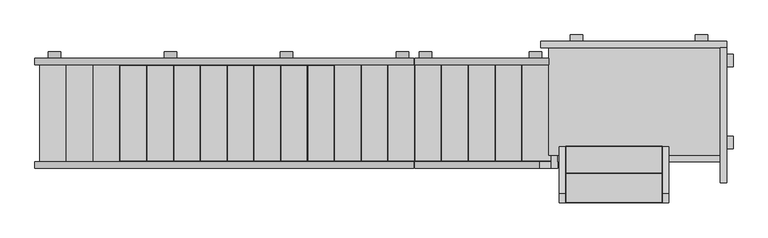
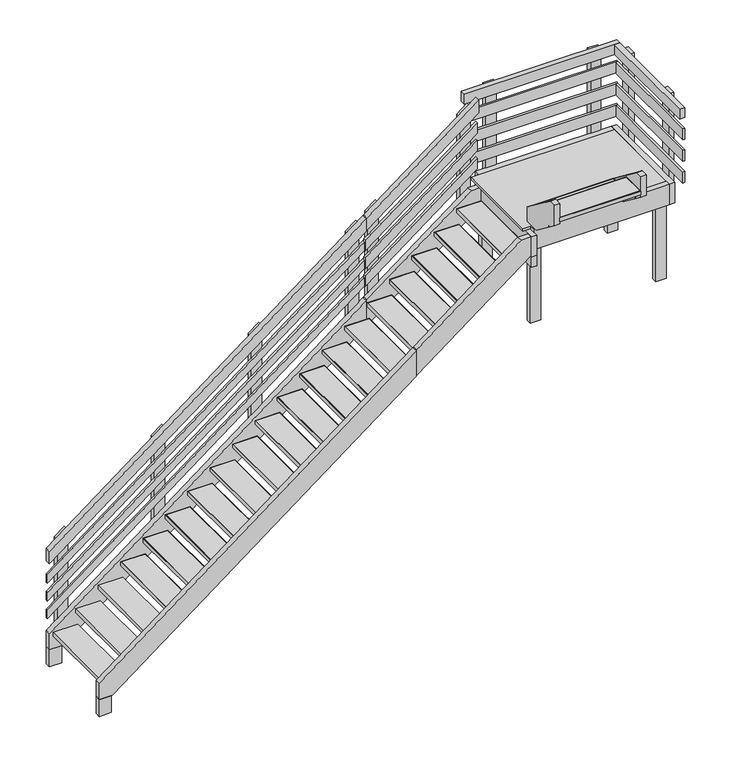
"""IFC4 building model written with IfcOpenShell, lengths in millimetres: stair geometry, Treppen : Treppen."""

from ifc_helpers import new_model, si_unit, frame, origin, place, context, project, spatial, polyline, outline, extrude, faceted_brep, source, transform, mapped, element, save


def stair_8a71ca67(model_context):
    return source(origin(), model_context, "Body", "SolidModel", [
        extrude(outline(polyline([(12040.927184, 9252.4494152), (12100.927184, 9252.4494152), (12100.927184, 9136.4494152), (12040.927184, 9136.4494152), (12040.927184, 9252.4494152)])), frame((0.0, 0.0, 3202.113), z_axis=(0.0, 0.0, 1.0), x_axis=(1.0, 0.0, 0.0)), (0.0, 0.0, 1.0), 1210.0),
        extrude(outline(polyline([(12040.927184, 10019.5272422), (12100.927184, 10019.5272422), (12100.927184, 9903.5272422), (12040.927184, 9903.5272422), (12040.927184, 10019.5272422)])), frame((0.0, 0.0, 3202.113), z_axis=(0.0, 0.0, 1.0), x_axis=(1.0, 0.0, 0.0)), (0.0, 0.0, 1.0), 1210.0),
        extrude(outline(polyline([(11748.927284, 10199.5272422), (11864.927284, 10199.5272422), (11864.927284, 10139.5272422), (11748.927284, 10139.5272422), (11748.927284, 10199.5272422)])), frame((0.0, 0.0, 3202.113), z_axis=(0.0, 0.0, 1.0), x_axis=(1.0, 0.0, 0.0)), (0.0, 0.0, 1.0), 1210.0),
        extrude(outline(polyline([(10580.970284, 10199.5272422), (10696.970284, 10199.5272422), (10696.970284, 10139.5272422), (10580.970284, 10139.5272422), (10580.970284, 10199.5272422)])), frame((0.0, 0.0, 3202.113), z_axis=(0.0, 0.0, 1.0), x_axis=(1.0, 0.0, 0.0)), (0.0, 0.0, 1.0), 1210.0),
        extrude(outline(polyline([(3061.4008007, 10198.6231113), (3149.5608007, 10314.6231113), (4355.2057254, 10314.6231113), (4267.0457213, 10198.6231113), (3061.4008007, 10198.6231113)])), frame((0.0, 9982.5272422, 0.0), z_axis=(0.0, 1.0, 0.0), x_axis=(0.0, 0.0, 1.0)), (0.0, 0.0, 1.0), 60.0),
        extrude(outline(polyline([(2282.7992976, 9174.1474494), (2370.9592976, 9290.1474494), (3576.6042224, 9290.1474494), (3488.4442183, 9174.1474494), (2282.7992976, 9174.1474494)])), frame((0.0, 9982.5272422, 0.0), z_axis=(0.0, 1.0, 0.0), x_axis=(0.0, 0.0, 1.0)), (0.0, 0.0, 1.0), 60.0),
        extrude(outline(polyline([(2118.4713054, 8957.926407), (2206.6313054, 9073.926407), (3412.2762301, 9073.926407), (3324.116226, 8957.926407), (2118.4713054, 8957.926407)])), frame((0.0, 9982.5272422, 0.0), z_axis=(0.0, 1.0, 0.0), x_axis=(0.0, 0.0, 1.0)), (0.0, 0.0, 1.0), 60.0),
        extrude(outline(polyline([(1295.3913054, 7874.926407), (1383.5513054, 7990.926407), (2589.1962301, 7990.926407), (2501.036226, 7874.926407), (1295.3913054, 7874.926407)])), frame((0.0, 9982.5272422, 0.0), z_axis=(0.0, 1.0, 0.0), x_axis=(0.0, 0.0, 1.0)), (0.0, 0.0, 1.0), 60.0),
        extrude(outline(polyline([(472.3113054, 6791.926407), (560.4713054, 6907.926407), (1766.1162301, 6907.926407), (1677.956226, 6791.926407), (472.3113054, 6791.926407)])), frame((0.0, 9982.5272422, 0.0), z_axis=(0.0, 1.0, 0.0), x_axis=(0.0, 0.0, 1.0)), (0.0, 0.0, 1.0), 60.0),
        extrude(outline(polyline([(-350.7686946, 5708.926407), (-262.6086946, 5824.926407), (943.036192, 5824.926407), (854.8761879, 5708.926407), (-350.7686946, 5708.926407)])), frame((0.0, 9982.5272422, 0.0), z_axis=(0.0, 1.0, 0.0), x_axis=(0.0, 0.0, 1.0)), (0.0, 0.0, 1.0), 60.0),
        extrude(outline(polyline([(12016.927184, 10115.5272422), (12040.927184, 10115.5272422), (12040.927184, 8819.5272422), (12016.927184, 8819.5272422), (12016.927184, 10115.5272422)])), frame((0.0, 0.0, 4072.113), z_axis=(0.0, 0.0, 1.0), x_axis=(1.0, 0.0, 0.0)), (0.0, 0.0, 1.0), 130.0),
        extrude(outline(polyline([(12016.927184, 10115.5272422), (12040.927184, 10115.5272422), (12040.927184, 8819.5272422), (12016.927184, 8819.5272422), (12016.927184, 10115.5272422)])), frame((0.0, 0.0, 3817.113), z_axis=(0.0, 0.0, 1.0), x_axis=(1.0, 0.0, 0.0)), (0.0, 0.0, 1.0), 130.0),
        extrude(outline(polyline([(12016.927184, 10115.5272422), (12040.927184, 10115.5272422), (12040.927184, 8819.5272422), (12016.927184, 8819.5272422), (12016.927184, 10115.5272422)])), frame((0.0, 0.0, 3562.113), z_axis=(0.0, 0.0, 1.0), x_axis=(1.0, 0.0, 0.0)), (0.0, 0.0, 1.0), 130.0),
        extrude(outline(polyline([(11980.927184, 10079.5272422), (12040.927184, 10079.5272422), (12040.927184, 8819.5272422), (11980.927184, 8819.5272422), (11980.927184, 10079.5272422)])), frame((0.0, 0.0, 4327.113), z_axis=(0.0, 0.0, 1.0), x_axis=(1.0, 0.0, 0.0)), (0.0, 0.0, 1.0), 116.0),
        extrude(outline(polyline([(10307.870484, 10139.5272422), (12040.927184, 10139.5272422), (12040.927184, 10115.5272422), (10307.870484, 10115.5272422), (10307.870484, 10139.5272422)])), frame((0.0, 0.0, 3562.113), z_axis=(0.0, 0.0, 1.0), x_axis=(1.0, 0.0, 0.0)), (0.0, 0.0, 1.0), 130.0),
        extrude(outline(polyline([(10307.870484, 10139.5272422), (12040.927184, 10139.5272422), (12040.927184, 10115.5272422), (10307.870484, 10115.5272422), (10307.870484, 10139.5272422)])), frame((0.0, 0.0, 3817.113), z_axis=(0.0, 0.0, 1.0), x_axis=(1.0, 0.0, 0.0)), (0.0, 0.0, 1.0), 130.0),
        extrude(outline(polyline([(10307.870484, 10139.5272422), (12040.927184, 10139.5272422), (12040.927184, 10115.5272422), (10307.870484, 10115.5272422), (10307.870484, 10139.5272422)])), frame((0.0, 0.0, 4072.113), z_axis=(0.0, 0.0, 1.0), x_axis=(1.0, 0.0, 0.0)), (0.0, 0.0, 1.0), 130.0),
        extrude(outline(polyline([(402.0866128, 5585.8451154), (3087.6090608, 9119.4271203), (3188.091099, 9119.4271181), (502.568651, 5585.8451132), (402.0866128, 5585.8451154)])), frame((0.0, 9958.5272422, 0.0), z_axis=(0.0, 1.0, 0.0), x_axis=(0.0, 0.0, 1.0)), (0.0, 0.0, 1.0), 24.0),
        extrude(outline(polyline([(2978.466099, 9119.4271181), (292.943651, 5585.8451132), (192.4616128, 5585.8451154), (2877.9840608, 9119.4271203), (2978.466099, 9119.4271181)])), frame((0.0, 9958.5272422, 0.0), z_axis=(0.0, 1.0, 0.0), x_axis=(0.0, 0.0, 1.0)), (0.0, 0.0, 1.0), 24.0),
        extrude(outline(polyline([(2768.841199, 9119.4271181), (83.318751, 5585.8451132), (-17.1632872, 5585.8451154), (2668.3591608, 9119.4271203), (2768.841199, 9119.4271181)])), frame((0.0, 9958.5272422, 0.0), z_axis=(0.0, 1.0, 0.0), x_axis=(0.0, 0.0, 1.0)), (0.0, 0.0, 1.0), 24.0),
        extrude(outline(polyline([(4158.2512383, 10379.427087), (3208.2512387, 9129.4271455), (3082.648691, 9129.4271483), (4032.6486905, 10379.4270898), (4158.2512383, 10379.427087)])), frame((0.0, 9958.5272422, 0.0), z_axis=(0.0, 1.0, 0.0), x_axis=(0.0, 0.0, 1.0)), (0.0, 0.0, 1.0), 24.0),
        extrude(outline(polyline([(3948.6263383, 10379.427087), (2998.6263387, 9129.4271455), (2873.023791, 9129.4271483), (3823.0237905, 10379.4270898), (3948.6263383, 10379.427087)])), frame((0.0, 9958.5272422, 0.0), z_axis=(0.0, 1.0, 0.0), x_axis=(0.0, 0.0, 1.0)), (0.0, 0.0, 1.0), 24.0),
        extrude(outline(polyline([(3739.0014383, 10379.427087), (2789.0014387, 9129.4271455), (2663.398891, 9129.4271483), (3613.3988905, 10379.4270898), (3739.0014383, 10379.427087)])), frame((0.0, 9958.5272422, 0.0), z_axis=(0.0, 1.0, 0.0), x_axis=(0.0, 0.0, 1.0)), (0.0, 0.0, 1.0), 24.0),
        extrude(outline(polyline([(10307.870484, 10139.5272422), (12040.927184, 10139.5272422), (12040.927184, 10079.5272422), (10307.870484, 10079.5272422), (10307.870484, 10139.5272422)])), frame((0.0, 0.0, 4327.113), z_axis=(0.0, 0.0, 1.0), x_axis=(1.0, 0.0, 0.0)), (0.0, 0.0, 1.0), 116.0),
        extrude(outline(polyline([(653.2916935, 5585.8451146), (3338.8141415, 9119.4271195), (3484.5130969, 9119.4271162), (798.9906489, 5585.8451113), (653.2916935, 5585.8451146)])), frame((0.0, 9922.5272422, 0.0), z_axis=(0.0, 1.0, 0.0), x_axis=(0.0, 0.0, 1.0)), (0.0, 0.0, 1.0), 60.0),
        extrude(outline(polyline([(3346.4144935, 9129.4272146), (4296.4144931, 10379.4271561), (4442.1134484, 10379.4271529), (3492.1134489, 9129.4272113), (3346.4144935, 9129.4272146)])), frame((0.0, 9922.5272422, 0.0), z_axis=(0.0, 1.0, 0.0), x_axis=(0.0, 0.0, 1.0)), (0.0, 0.0, 1.0), 60.0),
        extrude(outline(polyline([(11434.427184, 8904.5312493), (11434.427184, 8639.5272422), (10544.427184, 8639.5272422), (10544.427184, 8904.5312493), (11434.427184, 8904.5312493)])), frame((0.0, 0.0, 3777.5707232), z_axis=(0.0, 0.0, 1.0), x_axis=(1.0, 0.0, 0.0)), (0.0, 0.0, 1.0), 5.0),
        extrude(outline(polyline([(11439.427184, 8634.5272422), (10539.427184, 8634.5272422), (10539.427184, 8909.5312493), (11439.427184, 8909.5312493), (11439.427184, 8634.5272422)]), holes=[polyline([(11434.427184, 8639.5272422), (11434.427184, 8904.5312493), (10544.427184, 8904.5312493), (10544.427184, 8639.5272422), (11434.427184, 8639.5272422)])]), frame((0.0, 0.0, 3737.5707232), z_axis=(0.0, 0.0, 1.0), x_axis=(1.0, 0.0, 0.0)), (0.0, 0.0, 1.0), 45.0),
        extrude(outline(polyline([(11434.427184, 9154.5352565), (11434.427184, 8889.5312493), (10544.427184, 8889.5312493), (10544.427184, 9154.5352565), (11434.427184, 9154.5352565)])), frame((0.0, 0.0, 3607.113), z_axis=(0.0, 0.0, 1.0), x_axis=(1.0, 0.0, 0.0)), (0.0, 0.0, 1.0), 5.0),
        extrude(outline(polyline([(11439.427184, 8884.5312493), (10539.427184, 8884.5312493), (10539.427184, 9159.5352565), (11439.427184, 9159.5352565), (11439.427184, 8884.5312493)]), holes=[polyline([(11434.427184, 8889.5312493), (11434.427184, 9154.5352565), (10544.427184, 9154.5352565), (10544.427184, 8889.5312493), (11434.427184, 8889.5312493)])]), frame((0.0, 0.0, 3567.113), z_axis=(0.0, 0.0, 1.0), x_axis=(1.0, 0.0, 0.0)), (0.0, 0.0, 1.0), 45.0),
        faceted_brep([(6404.427184, 9019.5272422, 212.113), (6404.427184, 9919.5272422, 212.113), (6129.427184, 9919.5272422, 212.113), (6129.427184, 9019.5272422, 212.113), (6404.427184, 9019.5272422, 167.113), (6129.427184, 9019.5272422, 167.113), (6129.427184, 9919.5272422, 167.113), (6404.427184, 9919.5272422, 167.113), (6399.427184, 9024.5272422, 167.113), (6399.427184, 9914.5272422, 167.113), (6134.427184, 9914.5272422, 167.113), (6134.427184, 9024.5272422, 167.113), (6134.427184, 9024.5272422, 207.113), (6399.427184, 9024.5272422, 207.113), (6134.427184, 9914.5272422, 207.113), (6399.427184, 9914.5272422, 207.113)], [[[0, 1, 2, 3]], [[4, 5, 6, 7], [8, 9, 10, 11]], [[1, 0, 4, 7]], [[2, 1, 7, 6]], [[3, 2, 6, 5]], [[0, 3, 5, 4]], [[8, 11, 12, 13]], [[11, 10, 14, 12]], [[10, 9, 15, 14]], [[9, 8, 13, 15]], [[13, 12, 14, 15]]]),
        faceted_brep([(6154.427184, 9019.5272422, 22.113), (6154.427184, 9919.5272422, 22.113), (5879.427184, 9919.5272422, 22.113), (5879.427184, 9019.5272422, 22.113), (6154.427184, 9019.5272422, -22.887), (5879.427184, 9019.5272422, -22.887), (5879.427184, 9919.5272422, -22.887), (6154.427184, 9919.5272422, -22.887), (6149.427184, 9024.5272422, -22.887), (6149.427184, 9914.5272422, -22.887), (5884.427184, 9914.5272422, -22.887), (5884.427184, 9024.5272422, -22.887), (5884.427184, 9024.5272422, 17.113), (6149.427184, 9024.5272422, 17.113), (5884.427184, 9914.5272422, 17.113), (6149.427184, 9914.5272422, 17.113)], [[[0, 1, 2, 3]], [[4, 5, 6, 7], [8, 9, 10, 11]], [[1, 0, 4, 7]], [[2, 1, 7, 6]], [[3, 2, 6, 5]], [[0, 3, 5, 4]], [[8, 11, 12, 13]], [[11, 10, 14, 12]], [[10, 9, 15, 14]], [[9, 8, 13, 15]], [[13, 12, 14, 15]]]),
        faceted_brep([(5904.427184, 9019.5272422, -212.887), (5629.427184, 9019.5272422, -212.887), (5629.427184, 9919.5272422, -212.887), (5904.427184, 9919.5272422, -212.887), (5899.427184, 9024.5272422, -212.887), (5899.427184, 9914.5272422, -212.887), (5634.427184, 9914.5272422, -212.887), (5634.427184, 9024.5272422, -212.887), (5904.427184, 9919.5272422, -167.887), (5904.427184, 9019.5272422, -167.887), (5629.427184, 9919.5272422, -167.887), (5629.427184, 9019.5272422, -167.887), (5634.427184, 9024.5272422, -172.887), (5899.427184, 9024.5272422, -172.887), (5634.427184, 9914.5272422, -172.887), (5899.427184, 9914.5272422, -172.887)], [[[0, 1, 2, 3], [4, 5, 6, 7]], [[8, 9, 0, 3]], [[10, 8, 3, 2]], [[11, 10, 2, 1]], [[9, 11, 1, 0]], [[4, 7, 12, 13]], [[7, 6, 14, 12]], [[6, 5, 15, 14]], [[5, 4, 13, 15]], [[13, 12, 14, 15]], [[9, 8, 10, 11]]]),
        extrude(outline(polyline([(10399.427184, 9914.5272422), (10399.427184, 9024.5272422), (10134.427184, 9024.5272422), (10134.427184, 9914.5272422), (10399.427184, 9914.5272422)])), frame((0.0, 0.0, 3247.113), z_axis=(0.0, 0.0, 1.0), x_axis=(1.0, 0.0, 0.0)), (0.0, 0.0, 1.0), 5.0),
        extrude(outline(polyline([(10404.427184, 9019.5272422), (10129.427184, 9019.5272422), (10129.427184, 9919.5272422), (10404.427184, 9919.5272422), (10404.427184, 9019.5272422)]), holes=[polyline([(10399.427184, 9024.5272422), (10399.427184, 9914.5272422), (10134.427184, 9914.5272422), (10134.427184, 9024.5272422), (10399.427184, 9024.5272422)])]), frame((0.0, 0.0, 3207.113), z_axis=(0.0, 0.0, 1.0), x_axis=(1.0, 0.0, 0.0)), (0.0, 0.0, 1.0), 45.0),
        extrude(outline(polyline([(10149.427184, 9914.5272422), (10149.427184, 9024.5272422), (9884.427184, 9024.5272422), (9884.427184, 9914.5272422), (10149.427184, 9914.5272422)])), frame((0.0, 0.0, 3057.113), z_axis=(0.0, 0.0, 1.0), x_axis=(1.0, 0.0, 0.0)), (0.0, 0.0, 1.0), 5.0),
        extrude(outline(polyline([(10154.427184, 9019.5272422), (9879.427184, 9019.5272422), (9879.427184, 9919.5272422), (10154.427184, 9919.5272422), (10154.427184, 9019.5272422)]), holes=[polyline([(10149.427184, 9024.5272422), (10149.427184, 9914.5272422), (9884.427184, 9914.5272422), (9884.427184, 9024.5272422), (10149.427184, 9024.5272422)])]), frame((0.0, 0.0, 3017.113), z_axis=(0.0, 0.0, 1.0), x_axis=(1.0, 0.0, 0.0)), (0.0, 0.0, 1.0), 45.0),
        extrude(outline(polyline([(9899.427184, 9914.5272422), (9899.427184, 9024.5272422), (9634.427184, 9024.5272422), (9634.427184, 9914.5272422), (9899.427184, 9914.5272422)])), frame((0.0, 0.0, 2867.113), z_axis=(0.0, 0.0, 1.0), x_axis=(1.0, 0.0, 0.0)), (0.0, 0.0, 1.0), 5.0),
        extrude(outline(polyline([(9904.427184, 9019.5272422), (9629.427184, 9019.5272422), (9629.427184, 9919.5272422), (9904.427184, 9919.5272422), (9904.427184, 9019.5272422)]), holes=[polyline([(9899.427184, 9024.5272422), (9899.427184, 9914.5272422), (9634.427184, 9914.5272422), (9634.427184, 9024.5272422), (9899.427184, 9024.5272422)])]), frame((0.0, 0.0, 2827.113), z_axis=(0.0, 0.0, 1.0), x_axis=(1.0, 0.0, 0.0)), (0.0, 0.0, 1.0), 45.0),
        extrude(outline(polyline([(9649.427184, 9914.5272422), (9649.427184, 9024.5272422), (9384.427184, 9024.5272422), (9384.427184, 9914.5272422), (9649.427184, 9914.5272422)])), frame((0.0, 0.0, 2677.113), z_axis=(0.0, 0.0, 1.0), x_axis=(1.0, 0.0, 0.0)), (0.0, 0.0, 1.0), 5.0),
        extrude(outline(polyline([(9654.427184, 9019.5272422), (9379.427184, 9019.5272422), (9379.427184, 9919.5272422), (9654.427184, 9919.5272422), (9654.427184, 9019.5272422)]), holes=[polyline([(9649.427184, 9024.5272422), (9649.427184, 9914.5272422), (9384.427184, 9914.5272422), (9384.427184, 9024.5272422), (9649.427184, 9024.5272422)])]), frame((0.0, 0.0, 2637.113), z_axis=(0.0, 0.0, 1.0), x_axis=(1.0, 0.0, 0.0)), (0.0, 0.0, 1.0), 45.0),
        extrude(outline(polyline([(9399.427184, 9914.5272422), (9399.427184, 9024.5272422), (9134.427184, 9024.5272422), (9134.427184, 9914.5272422), (9399.427184, 9914.5272422)])), frame((0.0, 0.0, 2487.113), z_axis=(0.0, 0.0, 1.0), x_axis=(1.0, 0.0, 0.0)), (0.0, 0.0, 1.0), 5.0),
        extrude(outline(polyline([(9404.427184, 9019.5272422), (9129.427184, 9019.5272422), (9129.427184, 9919.5272422), (9404.427184, 9919.5272422), (9404.427184, 9019.5272422)]), holes=[polyline([(9399.427184, 9024.5272422), (9399.427184, 9914.5272422), (9134.427184, 9914.5272422), (9134.427184, 9024.5272422), (9399.427184, 9024.5272422)])]), frame((0.0, 0.0, 2447.113), z_axis=(0.0, 0.0, 1.0), x_axis=(1.0, 0.0, 0.0)), (0.0, 0.0, 1.0), 45.0),
        extrude(outline(polyline([(9149.427184, 9914.5272422), (9149.427184, 9024.5272422), (8884.427184, 9024.5272422), (8884.427184, 9914.5272422), (9149.427184, 9914.5272422)])), frame((0.0, 0.0, 2297.113), z_axis=(0.0, 0.0, 1.0), x_axis=(1.0, 0.0, 0.0)), (0.0, 0.0, 1.0), 5.0),
        extrude(outline(polyline([(9154.427184, 9019.5272422), (8879.427184, 9019.5272422), (8879.427184, 9919.5272422), (9154.427184, 9919.5272422), (9154.427184, 9019.5272422)]), holes=[polyline([(9149.427184, 9024.5272422), (9149.427184, 9914.5272422), (8884.427184, 9914.5272422), (8884.427184, 9024.5272422), (9149.427184, 9024.5272422)])]), frame((0.0, 0.0, 2257.113), z_axis=(0.0, 0.0, 1.0), x_axis=(1.0, 0.0, 0.0)), (0.0, 0.0, 1.0), 45.0),
        extrude(outline(polyline([(8899.427184, 9914.5272422), (8899.427184, 9024.5272422), (8634.427184, 9024.5272422), (8634.427184, 9914.5272422), (8899.427184, 9914.5272422)])), frame((0.0, 0.0, 2107.113), z_axis=(0.0, 0.0, 1.0), x_axis=(1.0, 0.0, 0.0)), (0.0, 0.0, 1.0), 5.0),
        extrude(outline(polyline([(8904.427184, 9019.5272422), (8629.427184, 9019.5272422), (8629.427184, 9919.5272422), (8904.427184, 9919.5272422), (8904.427184, 9019.5272422)]), holes=[polyline([(8899.427184, 9024.5272422), (8899.427184, 9914.5272422), (8634.427184, 9914.5272422), (8634.427184, 9024.5272422), (8899.427184, 9024.5272422)])]), frame((0.0, 0.0, 2067.113), z_axis=(0.0, 0.0, 1.0), x_axis=(1.0, 0.0, 0.0)), (0.0, 0.0, 1.0), 45.0),
        extrude(outline(polyline([(8649.427184, 9914.5272422), (8649.427184, 9024.5272422), (8384.427184, 9024.5272422), (8384.427184, 9914.5272422), (8649.427184, 9914.5272422)])), frame((0.0, 0.0, 1917.113), z_axis=(0.0, 0.0, 1.0), x_axis=(1.0, 0.0, 0.0)), (0.0, 0.0, 1.0), 5.0),
        extrude(outline(polyline([(8654.427184, 9019.5272422), (8379.427184, 9019.5272422), (8379.427184, 9919.5272422), (8654.427184, 9919.5272422), (8654.427184, 9019.5272422)]), holes=[polyline([(8649.427184, 9024.5272422), (8649.427184, 9914.5272422), (8384.427184, 9914.5272422), (8384.427184, 9024.5272422), (8649.427184, 9024.5272422)])]), frame((0.0, 0.0, 1877.113), z_axis=(0.0, 0.0, 1.0), x_axis=(1.0, 0.0, 0.0)), (0.0, 0.0, 1.0), 45.0),
        extrude(outline(polyline([(8399.427184, 9914.5272422), (8399.427184, 9024.5272422), (8134.427184, 9024.5272422), (8134.427184, 9914.5272422), (8399.427184, 9914.5272422)])), frame((0.0, 0.0, 1727.113), z_axis=(0.0, 0.0, 1.0), x_axis=(1.0, 0.0, 0.0)), (0.0, 0.0, 1.0), 5.0),
        extrude(outline(polyline([(8404.427184, 9019.5272422), (8129.427184, 9019.5272422), (8129.427184, 9919.5272422), (8404.427184, 9919.5272422), (8404.427184, 9019.5272422)]), holes=[polyline([(8399.427184, 9024.5272422), (8399.427184, 9914.5272422), (8134.427184, 9914.5272422), (8134.427184, 9024.5272422), (8399.427184, 9024.5272422)])]), frame((0.0, 0.0, 1687.113), z_axis=(0.0, 0.0, 1.0), x_axis=(1.0, 0.0, 0.0)), (0.0, 0.0, 1.0), 45.0),
        extrude(outline(polyline([(8149.427184, 9914.5272422), (8149.427184, 9024.5272422), (7884.427184, 9024.5272422), (7884.427184, 9914.5272422), (8149.427184, 9914.5272422)])), frame((0.0, 0.0, 1537.113), z_axis=(0.0, 0.0, 1.0), x_axis=(1.0, 0.0, 0.0)), (0.0, 0.0, 1.0), 5.0),
        extrude(outline(polyline([(8154.427184, 9019.5272422), (7879.427184, 9019.5272422), (7879.427184, 9919.5272422), (8154.427184, 9919.5272422), (8154.427184, 9019.5272422)]), holes=[polyline([(8149.427184, 9024.5272422), (8149.427184, 9914.5272422), (7884.427184, 9914.5272422), (7884.427184, 9024.5272422), (8149.427184, 9024.5272422)])]), frame((0.0, 0.0, 1497.113), z_axis=(0.0, 0.0, 1.0), x_axis=(1.0, 0.0, 0.0)), (0.0, 0.0, 1.0), 45.0),
        extrude(outline(polyline([(7899.427184, 9914.5272422), (7899.427184, 9024.5272422), (7634.427184, 9024.5272422), (7634.427184, 9914.5272422), (7899.427184, 9914.5272422)])), frame((0.0, 0.0, 1347.113), z_axis=(0.0, 0.0, 1.0), x_axis=(1.0, 0.0, 0.0)), (0.0, 0.0, 1.0), 5.0),
        extrude(outline(polyline([(7904.427184, 9019.5272422), (7629.427184, 9019.5272422), (7629.427184, 9919.5272422), (7904.427184, 9919.5272422), (7904.427184, 9019.5272422)]), holes=[polyline([(7899.427184, 9024.5272422), (7899.427184, 9914.5272422), (7634.427184, 9914.5272422), (7634.427184, 9024.5272422), (7899.427184, 9024.5272422)])]), frame((0.0, 0.0, 1307.113), z_axis=(0.0, 0.0, 1.0), x_axis=(1.0, 0.0, 0.0)), (0.0, 0.0, 1.0), 45.0),
        extrude(outline(polyline([(7649.427184, 9914.5272422), (7649.427184, 9024.5272422), (7384.427184, 9024.5272422), (7384.427184, 9914.5272422), (7649.427184, 9914.5272422)])), frame((0.0, 0.0, 1157.113), z_axis=(0.0, 0.0, 1.0), x_axis=(1.0, 0.0, 0.0)), (0.0, 0.0, 1.0), 5.0),
        extrude(outline(polyline([(7654.427184, 9019.5272422), (7379.427184, 9019.5272422), (7379.427184, 9919.5272422), (7654.427184, 9919.5272422), (7654.427184, 9019.5272422)]), holes=[polyline([(7649.427184, 9024.5272422), (7649.427184, 9914.5272422), (7384.427184, 9914.5272422), (7384.427184, 9024.5272422), (7649.427184, 9024.5272422)])]), frame((0.0, 0.0, 1117.113), z_axis=(0.0, 0.0, 1.0), x_axis=(1.0, 0.0, 0.0)), (0.0, 0.0, 1.0), 45.0),
        extrude(outline(polyline([(7399.427184, 9914.5272422), (7399.427184, 9024.5272422), (7134.427184, 9024.5272422), (7134.427184, 9914.5272422), (7399.427184, 9914.5272422)])), frame((0.0, 0.0, 967.113), z_axis=(0.0, 0.0, 1.0), x_axis=(1.0, 0.0, 0.0)), (0.0, 0.0, 1.0), 5.0),
        extrude(outline(polyline([(7404.427184, 9019.5272422), (7129.427184, 9019.5272422), (7129.427184, 9919.5272422), (7404.427184, 9919.5272422), (7404.427184, 9019.5272422)]), holes=[polyline([(7399.427184, 9024.5272422), (7399.427184, 9914.5272422), (7134.427184, 9914.5272422), (7134.427184, 9024.5272422), (7399.427184, 9024.5272422)])]), frame((0.0, 0.0, 927.113), z_axis=(0.0, 0.0, 1.0), x_axis=(1.0, 0.0, 0.0)), (0.0, 0.0, 1.0), 45.0),
        extrude(outline(polyline([(7149.427184, 9914.5272422), (7149.427184, 9024.5272422), (6884.427184, 9024.5272422), (6884.427184, 9914.5272422), (7149.427184, 9914.5272422)])), frame((0.0, 0.0, 777.113), z_axis=(0.0, 0.0, 1.0), x_axis=(1.0, 0.0, 0.0)), (0.0, 0.0, 1.0), 5.0),
        extrude(outline(polyline([(7154.427184, 9019.5272422), (6879.427184, 9019.5272422), (6879.427184, 9919.5272422), (7154.427184, 9919.5272422), (7154.427184, 9019.5272422)]), holes=[polyline([(7149.427184, 9024.5272422), (7149.427184, 9914.5272422), (6884.427184, 9914.5272422), (6884.427184, 9024.5272422), (7149.427184, 9024.5272422)])]), frame((0.0, 0.0, 737.113), z_axis=(0.0, 0.0, 1.0), x_axis=(1.0, 0.0, 0.0)), (0.0, 0.0, 1.0), 45.0),
        extrude(outline(polyline([(6899.427184, 9914.5272422), (6899.427184, 9024.5272422), (6634.427184, 9024.5272422), (6634.427184, 9914.5272422), (6899.427184, 9914.5272422)])), frame((0.0, 0.0, 587.113), z_axis=(0.0, 0.0, 1.0), x_axis=(1.0, 0.0, 0.0)), (0.0, 0.0, 1.0), 5.0),
        extrude(outline(polyline([(6904.427184, 9019.5272422), (6629.427184, 9019.5272422), (6629.427184, 9919.5272422), (6904.427184, 9919.5272422), (6904.427184, 9019.5272422)]), holes=[polyline([(6899.427184, 9024.5272422), (6899.427184, 9914.5272422), (6634.427184, 9914.5272422), (6634.427184, 9024.5272422), (6899.427184, 9024.5272422)])]), frame((0.0, 0.0, 547.113), z_axis=(0.0, 0.0, 1.0), x_axis=(1.0, 0.0, 0.0)), (0.0, 0.0, 1.0), 45.0),
        extrude(outline(polyline([(6649.427184, 9914.5272422), (6649.427184, 9024.5272422), (6384.427184, 9024.5272422), (6384.427184, 9914.5272422), (6649.427184, 9914.5272422)])), frame((0.0, 0.0, 397.113), z_axis=(0.0, 0.0, 1.0), x_axis=(1.0, 0.0, 0.0)), (0.0, 0.0, 1.0), 5.0),
        extrude(outline(polyline([(6654.427184, 9019.5272422), (6379.427184, 9019.5272422), (6379.427184, 9919.5272422), (6654.427184, 9919.5272422), (6654.427184, 9019.5272422)]), holes=[polyline([(6649.427184, 9024.5272422), (6649.427184, 9914.5272422), (6384.427184, 9914.5272422), (6384.427184, 9024.5272422), (6649.427184, 9024.5272422)])]), frame((0.0, 0.0, 357.113), z_axis=(0.0, 0.0, 1.0), x_axis=(1.0, 0.0, 0.0)), (0.0, 0.0, 1.0), 45.0),
        faceted_brep([(11977.927184, 9078.0272422, 3442.113), (11977.927184, 10078.0272422, 3442.113), (10380.927184, 10078.0272422, 3442.113), (10380.927184, 9078.0272422, 3442.113), (11977.927184, 9078.0272422, 3410.113), (10380.927184, 9078.0272422, 3410.113), (10380.927184, 10078.0272422, 3410.113), (11977.927184, 10078.0272422, 3410.113), (11972.927184, 9083.0272422, 3410.113), (11972.927184, 10073.0272422, 3410.113), (10385.927184, 10073.0272422, 3410.113), (10385.927184, 9083.0272422, 3410.113), (10385.927184, 9083.0272422, 3437.1), (11972.927184, 9083.0272422, 3437.1), (10385.927184, 10073.0272422, 3437.1), (11972.927184, 10073.0272422, 3437.1)], [[[0, 1, 2, 3]], [[4, 5, 6, 7], [8, 9, 10, 11]], [[1, 0, 4, 7]], [[2, 1, 7, 6]], [[3, 2, 6, 5]], [[0, 3, 5, 4]], [[8, 11, 12, 13]], [[11, 10, 14, 12]], [[10, 9, 15, 14]], [[9, 8, 13, 15]], [[13, 12, 14, 15]]]),
        extrude(outline(polyline([(10404.427184, 9019.5272422), (10129.427184, 9019.5272422), (10129.427184, 9919.5272422), (10404.427184, 9919.5272422), (10404.427184, 9019.5272422)]), holes=[polyline([(10399.427184, 9024.5272422), (10399.427184, 9914.5272422), (10134.427184, 9914.5272422), (10134.427184, 9024.5272422), (10399.427184, 9024.5272422)])]), frame((0.0, 0.0, 3207.113), z_axis=(0.0, 0.0, 1.0), x_axis=(1.0, 0.0, 0.0)), (0.0, 0.0, 1.0), 45.0),
        extrude(outline(polyline([(8754.5272422, 3618.9858282), (8754.5272422, 3650.0), (8713.7144763, 3650.0), (8634.5272422, 3710.1754483), (8634.5272422, 3950.0), (8715.5589191, 3950.0), (9154.5155135, 3616.4309577), (9154.5155135, 3442.113), (8987.2811385, 3442.113), (8754.5272422, 3618.9858282)])), frame((10476.427184, 0.0, 0.0), z_axis=(1.0, 0.0, 0.0), x_axis=(0.0, 1.0, 0.0)), (0.0, 0.0, 1.0), 60.0),
        extrude(outline(polyline([(8754.5272422, 3618.9858282), (8754.5272422, 3650.0), (8713.7144763, 3650.0), (8634.5272422, 3710.1754483), (8634.5272422, 3950.0), (8715.5589191, 3950.0), (9154.5155135, 3616.4309577), (9154.5155135, 3442.113), (8987.2811385, 3442.113), (8754.5272422, 3618.9858282)])), frame((11442.427184, 0.0, 0.0), z_axis=(1.0, 0.0, 0.0), x_axis=(0.0, 1.0, 0.0)), (0.0, 0.0, 1.0), 60.0),
        extrude(outline(polyline([(10464.970284, 9076.5272422), (11980.927184, 9076.5272422), (11980.927184, 9016.5272422), (10464.970284, 9016.5272422), (10464.970284, 9076.5272422)])), frame((0.0, 0.0, 3202.113), z_axis=(0.0, 0.0, 1.0), x_axis=(1.0, 0.0, 0.0)), (0.0, 0.0, 1.0), 240.0),
        extrude(outline(polyline([(10464.970284, 10139.5272422), (11980.927184, 10139.5272422), (11980.927184, 10079.5272422), (10464.970284, 10079.5272422), (10464.970284, 10139.5272422)])), frame((0.0, 0.0, 3202.113), z_axis=(0.0, 0.0, 1.0), x_axis=(1.0, 0.0, 0.0)), (0.0, 0.0, 1.0), 240.0),
        extrude(outline(polyline([(2295.0, 11864.927284), (2295.0, 11980.927284), (3330.113, 11980.927284), (3330.113, 11956.927284), (3410.113, 11956.927284), (3410.113, 11864.927284), (2295.0, 11864.927284)])), frame((0.0, 10019.5272422, 0.0), z_axis=(0.0, 1.0, 0.0), x_axis=(0.0, 0.0, 1.0)), (0.0, 0.0, 1.0), 60.0),
        extrude(outline(polyline([(11980.927184, 10139.5272422), (12040.927184, 10139.5272422), (12040.927184, 9016.5272422), (11980.927184, 9016.5272422), (11980.927184, 10139.5272422)])), frame((0.0, 0.0, 3202.113), z_axis=(0.0, 0.0, 1.0), x_axis=(1.0, 0.0, 0.0)), (0.0, 0.0, 1.0), 240.0),
        extrude(outline(polyline([(11956.927284, 10079.5272422), (11980.927284, 10079.5272422), (11980.927284, 9076.5272422), (11956.927284, 9076.5272422), (11956.927284, 10079.5272422)])), frame((0.0, 0.0, 3330.113), z_axis=(0.0, 0.0, 1.0), x_axis=(1.0, 0.0, 0.0)), (0.0, 0.0, 1.0), 80.0),
        extrude(outline(polyline([(2295.0, 11864.927284), (2295.0, 11980.927284), (3330.113, 11980.927284), (3330.113, 11956.927284), (3410.113, 11956.927284), (3410.113, 11864.927284), (2295.0, 11864.927284)])), frame((0.0, 9076.5272422, 0.0), z_axis=(0.0, 1.0, 0.0), x_axis=(0.0, 0.0, 1.0)), (0.0, 0.0, 1.0), 60.0),
        extrude(outline(polyline([(10464.970284, 10079.5272422), (10488.970284, 10079.5272422), (10488.970284, 9076.5272422), (10464.970284, 9076.5272422), (10464.970284, 10079.5272422)])), frame((0.0, 0.0, 3330.113), z_axis=(0.0, 0.0, 1.0), x_axis=(1.0, 0.0, 0.0)), (0.0, 0.0, 1.0), 80.0),
        extrude(outline(polyline([(2295.0, 10580.970284), (3410.113, 10580.970284), (3410.113, 10488.970284), (3330.113, 10488.970284), (3330.113, 10464.970284), (2295.0, 10464.970284), (2295.0, 10580.970284)])), frame((0.0, 9076.5272422, 0.0), z_axis=(0.0, 1.0, 0.0), x_axis=(0.0, 0.0, 1.0)), (0.0, 0.0, 1.0), 60.0),
        extrude(outline(polyline([(2295.0, 10580.970284), (3410.113, 10580.970284), (3410.113, 10488.970284), (3330.113, 10488.970284), (3330.113, 10464.970284), (2295.0, 10464.970284), (2295.0, 10580.970284)])), frame((0.0, 10019.5272422, 0.0), z_axis=(0.0, 1.0, 0.0), x_axis=(0.0, 0.0, 1.0)), (0.0, 0.0, 1.0), 60.0),
        extrude(outline(polyline([(10404.970284, 10140.0272422), (10464.970284, 10140.0272422), (10464.970284, 8956.5272422), (10404.970284, 8956.5272422), (10404.970284, 10140.0272422)])), frame((0.0, 0.0, 3048.113), z_axis=(0.0, 0.0, 1.0), x_axis=(1.0, 0.0, 0.0)), (0.0, 0.0, 1.0), 120.0),
        extrude(outline(polyline([(10404.970284, 9982.5272422), (10464.970284, 9982.5272422), (10464.970284, 8956.5272422), (10404.970284, 8956.5272422), (10404.970284, 9982.5272422)])), frame((0.0, 0.0, 3168.113), z_axis=(0.0, 0.0, 1.0), x_axis=(1.0, 0.0, 0.0)), (0.0, 0.0, 1.0), 240.0),
        extrude(outline(polyline([(5585.8451291, 9982.5272422), (5725.845084, 9982.5272422), (5725.845084, 9922.5272422), (5585.8451291, 9922.5272422), (5585.8451291, 9982.5272422)])), frame((0.0, 0.0, -560.9044), z_axis=(0.0, 0.0, 1.0), x_axis=(1.0, 0.0, 0.0)), (0.0, 0.0, 1.0), 200.0),
        extrude(outline(polyline([(5585.8451291, 9016.5272422), (5721.7556228, 9016.5272422), (5721.7556228, 8956.5272422), (5585.8451291, 8956.5272422), (5585.8451291, 9016.5272422)])), frame((0.0, 0.0, -560.9044), z_axis=(0.0, 0.0, 1.0), x_axis=(1.0, 0.0, 0.0)), (0.0, 0.0, 1.0), 200.0),
        extrude(outline(polyline([(-167.8643512, 5585.8451291), (-360.9044, 5585.8451291), (-360.9044, 5728.4846894), (2216.2220237, 9119.44051), (2517.6681382, 9119.44051), (-167.8643512, 5585.8451291)])), frame((0.0, 8956.5272422, 0.0), z_axis=(0.0, 1.0, 0.0), x_axis=(0.0, 0.0, 1.0)), (0.0, 0.0, 1.0), 60.0),
        extrude(outline(polyline([(3408.113, 10291.078486), (2525.2681382, 9129.44051), (2223.8220237, 9129.44051), (3193.2246519, 10404.970284), (3408.113, 10404.970284), (3408.113, 10291.078486)])), frame((0.0, 8956.5272422, 0.0), z_axis=(0.0, 1.0, 0.0), x_axis=(0.0, 0.0, 1.0)), (0.0, 0.0, 1.0), 60.0),
        extrude(outline(polyline([(-167.8643512, 5585.8451291), (-360.9044, 5585.8451291), (-360.9044, 5728.4846894), (2216.2220237, 9119.44051), (2517.6681382, 9119.44051), (-167.8643512, 5585.8451291)])), frame((0.0, 9922.5272422, 0.0), z_axis=(0.0, 1.0, 0.0), x_axis=(0.0, 0.0, 1.0)), (0.0, 0.0, 1.0), 60.0),
        extrude(outline(polyline([(3408.113, 10291.078486), (2525.2681382, 9129.44051), (2223.8220237, 9129.44051), (3193.2246519, 10404.970284), (3408.113, 10404.970284), (3408.113, 10291.078486)])), frame((0.0, 9922.5272422, 0.0), z_axis=(0.0, 1.0, 0.0), x_axis=(0.0, 0.0, 1.0)), (0.0, 0.0, 1.0), 60.0),
    ])


if __name__ == "__main__":
    model = new_model("IFC4")
    model_context = context("Model", 3, world=origin())
    ifc_project = project(units=[si_unit("LENGTHUNIT", "METRE", prefix="MILLI")], contexts=[model_context])
    site = spatial("IfcSite", under=ifc_project)
    building = spatial("IfcBuilding", under=site)
    placement = place(None, origin())
    stair_shape = stair_8a71ca67(model_context)
    element("IfcStair", 1, ObjectType="Treppen : Treppen", at=placement, inside=building, context=model_context, shape_type="MappedRepresentation", body=[
        mapped(stair_shape, transform((0.0, 0.0, 0.0), x_axis=(1.0, 0.0, 0.0), y_axis=(0.0, 1.0, 0.0), z_axis=(0.0, 0.0, 1.0))),
    ])
    save(model, "model.ifc")

# Revit data of these elements
# Type "Treppen : Treppen"
#   Material Stufen [instance default] = Metall - Baustahl S235
#   Material Wangen [instance default] = Holz - C 20 Cl.1
#   Material Geländer Stützen Podest [instance default] = Holz - C 20 Cl.1
#   Material Auflager [instance default] = Holz - C 20 Cl.1
# Element 1 (IfcStair, "Treppen : Treppen")
#   Materials on its faces: "Metall - Baustahl S235", "Holz - C 20 Cl.1"
# Materials
#   "Metall - Baustahl S235": class "Metall", colour RGB 159 159 159, transparency 0, Description = "Baustahl S235", Cost = 0
#   "Holz - C 20 Cl.1": class "Holz", colour RGB 218 191 173, transparency 0, Description = "Holz - C 20 Cl.1", Cost = 0
